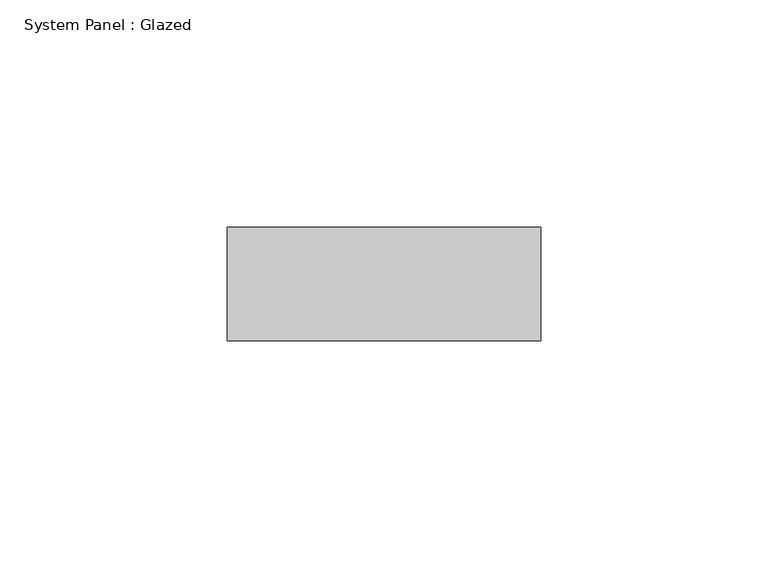
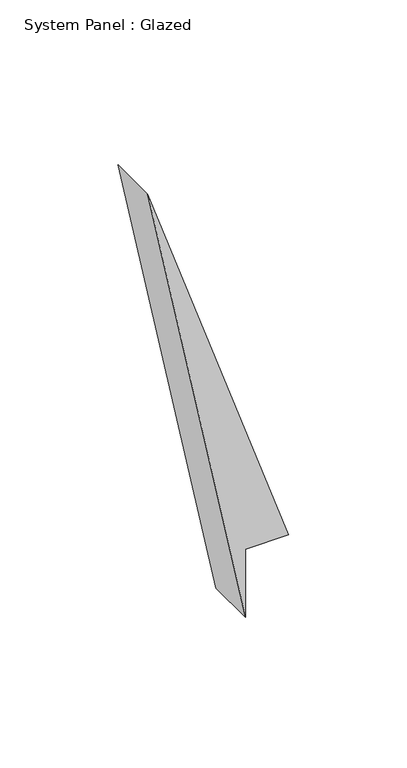
"""IFC4 building model written with IfcOpenShell, lengths in millimetres: plate geometry, System Panel : Glazed."""

from ifc_helpers import new_model, si_unit, frame, origin, place, context, project, spatial, polyline, outline, extrude, source, transform, mapped, element, save


def system_panel_glazed_d456bf06(model_context):
    return source(origin(), model_context, "Body", "SweptSolid", [
        extrude(outline(polyline([(0.0, 13.3598871), (35.3553391, 13.3598871), (35.3553391, 34.5595931), (235.5726611, -34.5595931), (0.0, 13.3598871)])), frame((0.0, -49.5, 0.0), z_axis=(0.0, 1.0, 0.0), x_axis=(0.0, 0.0, 1.0)), (0.0, 0.0, 1.0), 25.0),
    ])


if __name__ == "__main__":
    model = new_model("IFC4")
    model_context = context("Model", 3, world=origin())
    ifc_project = project(units=[si_unit("LENGTHUNIT", "METRE", prefix="MILLI")], contexts=[model_context])
    site = spatial("IfcSite", under=ifc_project)
    building = spatial("IfcBuilding", under=site)
    placement = place(None, origin())
    system_panel_glazed_shape = system_panel_glazed_d456bf06(model_context)
    element("IfcPlate", 1, ObjectType="System Panel : Glazed", at=placement, inside=building, context=model_context, shape_type="MappedRepresentation", body=[
        mapped(system_panel_glazed_shape, transform((0.0, 0.0, 0.0), x_axis=(1.0, 0.0, 0.0), y_axis=(0.0, 1.0, 0.0), z_axis=(0.0, 0.0, 1.0))),
    ])
    save(model, "model.ifc")

# Revit data of these elements
# Element 1 (IfcPlate, "System Panel : Glazed")
#   Materials on its faces: "Glass"
# Materials
#   "Glass": class "Glass", colour RGB 218 227 224, transparency 0.85, Description = "Soda Lime Glass", Cost = 0
